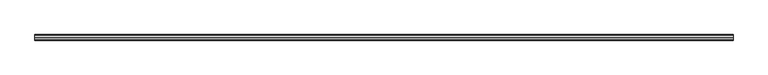
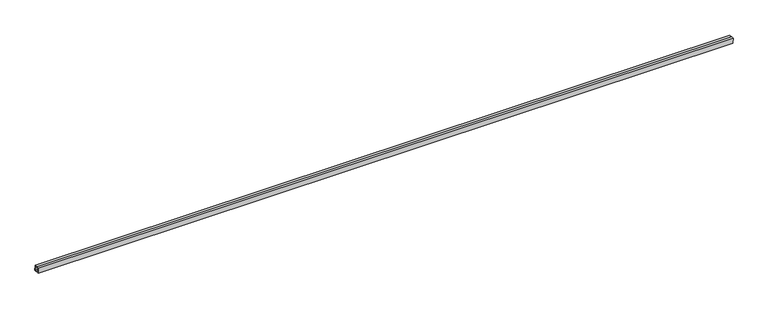
"""IFC4 building model written with IfcOpenShell, lengths in millimetres: proxy geometry, Inner panel:Inner panel:1:Inner panel:1 : Inner panel:Inner panel:300324:2:Inner panel:1:Inner panel:1 : Inner panel:Inner panel:300324:2 : Inner panel:Inner panel:1:Inner panel:1 : Inner panel:Inner panel:300324:300043:46 : Inner panel:Inner panel:1:Inner panel:1 : Inner panel:Inner panel:300324:2:Inner panel:1:Inner panel:1 : Inner panel:Inner panel:300324:2 : Inner panel:Inner panel:1:Inner panel:1 : Inner panel:Inner panel:300324:300043:308120."""

from ifc_helpers import new_model, si_unit, frame, origin, place, context, project, spatial, polyline, outline, extrude, source, transform, mapped, element, save


def generic_models_ed33f9ee(model_context):
    return source(origin(), model_context, "Body", "SweptSolid", [
        extrude(outline(polyline([(-577258.3887241, 4022.4942957), (-577240.148301, 4023.2543133), (-577238.5621772, 3985.1873432), (-577276.6291473, 3983.6012194), (-577278.215271, 4021.6681895), (-577259.9748479, 4022.4282072), (-577259.8757151, 4020.0490215), (-577275.7369527, 4019.3881366), (-577274.3490944, 3986.0795378), (-577241.0404956, 3987.4673961), (-577242.4283539, 4020.7759949), (-577258.2895914, 4020.11511), (-577258.3887241, 4022.4942957)])), frame((607854.1367239, 0.0, 0.0), z_axis=(1.0, 0.0, 0.0), x_axis=(0.0, 1.0, 0.0)), (0.0, 0.0, 1.0), 4876.8),
    ])


if __name__ == "__main__":
    model = new_model("IFC4")
    model_context = context("Model", 3, world=origin())
    ifc_project = project(units=[si_unit("LENGTHUNIT", "METRE", prefix="MILLI")], contexts=[model_context])
    site = spatial("IfcSite", under=ifc_project)
    building = spatial("IfcBuilding", under=site)
    placement = place(None, origin())
    generic_models_shape = generic_models_ed33f9ee(model_context)
    element("IfcBuildingElementProxy", 1, Name="Inner panel:Inner panel:1:Inner panel:1 : Inner panel:Inner panel:300324:2:Inner panel:1:Inner panel:1 : Inner panel:Inner panel:300324:2 : Inner panel:Inner panel:1:Inner panel:1 : Inner panel:Inner panel:300324:300043:46 : Inner panel:Inner panel:1:Inner panel:1 : Inner panel:Inner panel:300324:2:Inner panel:1:Inner panel:1 : Inner panel:Inner panel:300324:2 : Inner panel:Inner panel:1:Inner panel:1 : Inner panel:Inner panel:300324:300043:308120", ObjectType="Inner panel:Inner panel:1:Inner panel:1 : Inner panel:Inner panel:300324:2:Inner panel:1:Inner panel:1 : Inner panel:Inner panel:300324:2 : Inner panel:Inner panel:1:Inner panel:1 : Inner panel:Inner panel:300324:300043:46 : Inner panel:Inner panel:1:Inner panel:1 : Inner panel:Inner panel:300324:2:Inner panel:1:Inner panel:1 : Inner panel:Inner panel:300324:2 : Inner panel:Inner panel:1:Inner panel:1 : Inner panel:Inner panel:300324:300043:308120", at=placement, inside=building, context=model_context, shape_type="MappedRepresentation", body=[
        mapped(generic_models_shape, transform((0.0, 0.0, 0.0), x_axis=(1.0, 0.0, 0.0), y_axis=(0.0, 1.0, 0.0), z_axis=(0.0, 0.0, 1.0))),
    ])
    save(model, "model.ifc")

# Revit data of these elements
# Type "Inner panel:Inner panel:1:Inner panel:1 : Inner panel:Inner panel:300324:2:Inner panel:1:Inner panel:1 : Inner panel:Inner panel:300324:2 : Inner panel:Inner panel:1:Inner panel:1 : Inner panel:Inner panel:300324:300043:46 : Inner panel:Inner panel:1:Inner panel:1 : Inner panel:Inner panel:300324:2:Inner panel:1:Inner panel:1 : Inner panel:Inner panel:300324:2 : Inner panel:Inner panel:1:Inner panel:1 : Inner panel:Inner panel:300324:300043:308120"
#   NameOverride = "Inner panel:Inner panel:1:Inner panel:1 : Inner panel:Inner panel:300324:2:Inner panel:1:Inner panel:1 : Inner panel:Inner panel:300324:2 : Inner panel:Inner panel:1:Inner panel:1 : Inner panel:Inner panel:300324:300043:308120"
#   ObjectTypeOverride = "Inner panel:1:Inner panel:1 : Inner panel:Inner panel:300324:2 : Inner panel:Inner panel:1:Inner panel:1 : Inner panel:Inner panel:300324:300043"
#   Reference = "Inner panel"
#   Tag = "308120"
# Element 1 (IfcBuildingElementProxy, "Inner panel:Inner panel:1:Inner panel:1 : Inner panel:Inner panel:300324:2:Inner panel:1:Inner panel:1 : Inner panel:Inner panel:300324:2 : Inner panel:Inner panel:1:Inner panel:1 : Inner panel:Inner panel:300324:300043:46 : Inner panel:Inner panel:1:Inner panel:1 : Inner panel:Inner panel:300324:2:Inner panel:1:Inner panel:1 : Inner panel:Inner panel:300324:2 : Inner panel:Inner panel:1:Inner panel:1 : Inner panel:Inner panel:300324:300043:308120")
#   Materials on its faces: "1 1/2\" X 1 1/2\" SPLIT-SEAM SQUARE TUBING (~24\" CANTILEVER FROM C.L. OF GLULAM)"
# Materials
#   "1 1/2\" X 1 1/2\" SPLIT-SEAM SQUARE TUBING (~24\" CANTILEVER FROM C.L. OF GLULAM)": class "Unassigned", colour RGB 202 201 200, transparency 0, Cost = 0
